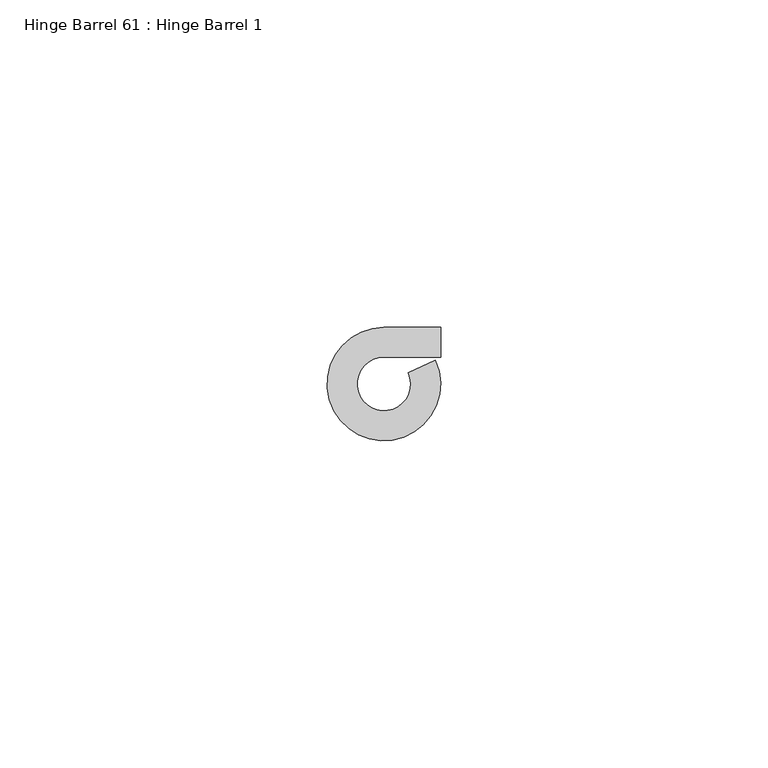
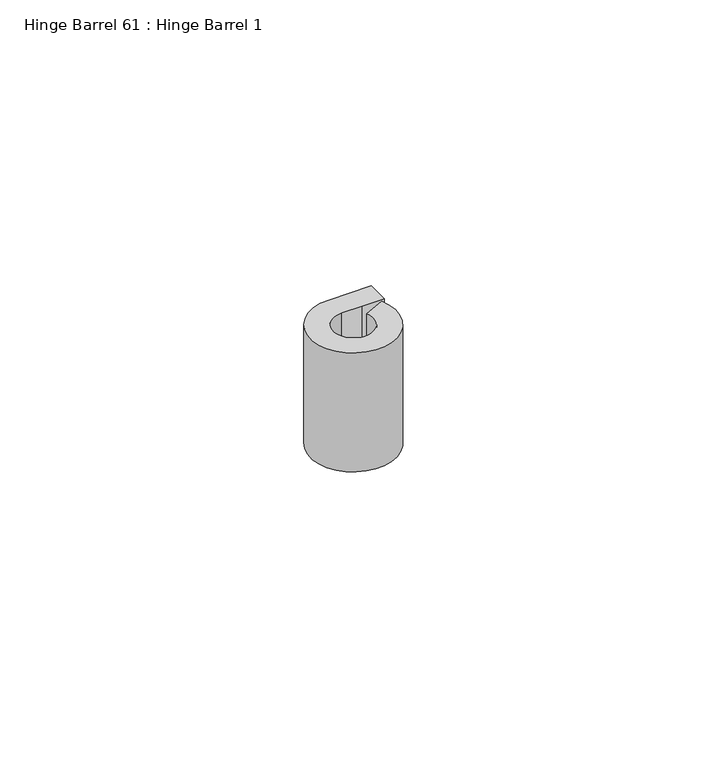
"""IFC4 building model written with IfcOpenShell, lengths in millimetres: proxy geometry, Hinge Barrel 61 : Hinge Barrel 1."""

from ifc_helpers import new_model, si_unit, point, frame, frame_2d, origin, place, context, project, spatial, polyline, circle_curve, trimmed, segment, composite_curve, outline, extrude, source, transform, mapped, element, save


def hinge_barrel_61_hinge_barrel_1_56b842ac(model_context):
    return source(origin(), model_context, "Body", "SweptSolid", [
        extrude(outline(composite_curve([segment(polyline([(587323.2214739, -536306.2758841), (587319.1320739, -536306.2758841)]), True, "CONTINUOUS"), segment(trimmed(circle_curve(frame_2d((587319.1320739, -536310.3652841)), 4.0894), [point((587319.1320739, -536306.2758841))], [point((587322.8436736, -536308.6485371))], True, "CARTESIAN"), True, "CONTINUOUS"), segment(polyline([(587322.8436736, -536308.6485371), (587326.986084, -536306.7325249)]), True, "CONTINUOUS"), segment(trimmed(circle_curve(frame_2d((587319.1320739, -536310.3652841)), 8.6534625), [point((587326.986084, -536306.7325249))], [point((587319.1320739, -536301.7118216))], False, "CARTESIAN"), True, "CONTINUOUS"), segment(polyline([(587319.1320739, -536301.7118216), (587327.7934739, -536301.7118216), (587327.7934739, -536306.2758841), (587323.2214739, -536306.2758841)]), True, "CONTINUOUS")], self_intersect=False)), frame((0.0, 0.0, 1936.75), z_axis=(0.0, 0.0, 1.0), x_axis=(1.0, 0.0, 0.0)), (0.0, 0.0, 1.0), 25.4),
    ])


if __name__ == "__main__":
    model = new_model("IFC4")
    model_context = context("Model", 3, world=origin())
    ifc_project = project(units=[si_unit("LENGTHUNIT", "METRE", prefix="MILLI")], contexts=[model_context])
    site = spatial("IfcSite", under=ifc_project)
    building = spatial("IfcBuilding", under=site)
    placement = place(None, origin())
    hinge_barrel_61_hinge_barrel_1_shape = hinge_barrel_61_hinge_barrel_1_56b842ac(model_context)
    element("IfcBuildingElementProxy", 1, Name="Hinge Barrel 61 : Hinge Barrel 1", ObjectType="Hinge Barrel 61 : Hinge Barrel 1", at=placement, inside=building, context=model_context, shape_type="MappedRepresentation", body=[
        mapped(hinge_barrel_61_hinge_barrel_1_shape, transform((0.0, 0.0, 0.0), x_axis=(1.0, 0.0, 0.0), y_axis=(0.0, 1.0, 0.0), z_axis=(0.0, 0.0, 1.0))),
    ])
    save(model, "model.ifc")

# Revit data of these elements
# Element 1 (IfcBuildingElementProxy, "Hinge Barrel 61 : Hinge Barrel 1")
#   Materials on its faces: "6\"X6\" WELD-ON STL BUTT HINGE"
# Materials
#   "6\"X6\" WELD-ON STL BUTT HINGE": class "Metal", colour RGB 189 187 185, transparency 0, Description = "Carbon steel", Cost = 0
